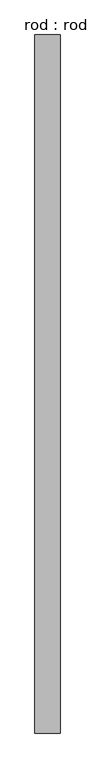
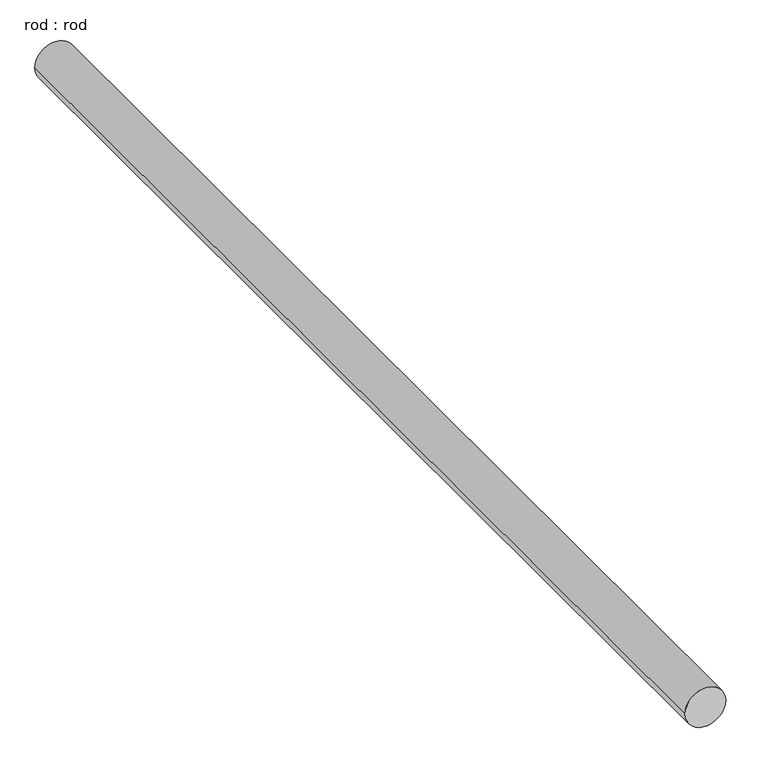
"""IFC4 building model written with IfcOpenShell, lengths in millimetres: proxy geometry, rod : rod."""

from ifc_helpers import new_model, si_unit, point, frame, frame_2d, origin, place, context, project, spatial, circle_curve, trimmed, segment, composite_curve, outline, extrude, source, transform, mapped, element, save


def rod_rod_ef537965(model_context):
    return source(origin(), model_context, "Body", "SweptSolid", [
        extrude(outline(composite_curve([segment(trimmed(circle_curve(frame_2d((0.0108462, 0.0)), 200.0), [point((0.0108462, 200.0))], [point((0.0108462, -200.0))], False, "CARTESIAN"), True, "CONTINUOUS"), segment(trimmed(circle_curve(frame_2d((0.0108462, 0.0)), 200.0), [point((0.0108462, -200.0))], [point((0.0108462, 200.0))], False, "CARTESIAN"), True, "CONTINUOUS")], self_intersect=False)), frame((0.0, -1457.2713847, 0.0), z_axis=(0.0, 1.0, 0.0), x_axis=(0.0, 0.0, 1.0)), (0.0, 0.0, 1.0), 11100.0),
    ])


if __name__ == "__main__":
    model = new_model("IFC4")
    model_context = context("Model", 3, world=origin())
    ifc_project = project(units=[si_unit("LENGTHUNIT", "METRE", prefix="MILLI")], contexts=[model_context])
    site = spatial("IfcSite", under=ifc_project)
    building = spatial("IfcBuilding", under=site)
    placement = place(None, origin())
    rod_rod_shape = rod_rod_ef537965(model_context)
    element("IfcBuildingElementProxy", 1, Name="rod : rod", ObjectType="rod : rod", at=placement, inside=building, context=model_context, shape_type="MappedRepresentation", body=[
        mapped(rod_rod_shape, transform((0.0, 0.0, 0.0), x_axis=(1.0, 0.0, 0.0), y_axis=(0.0, 1.0, 0.0), z_axis=(0.0, 0.0, 1.0))),
    ])
    save(model, "model.ifc")

# Revit data of these elements
# Type "rod : rod"
#   Default Elevation = 0
